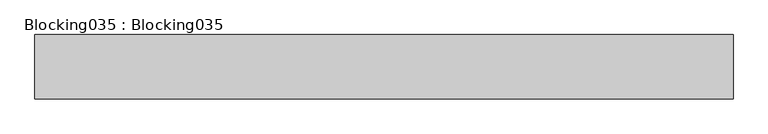
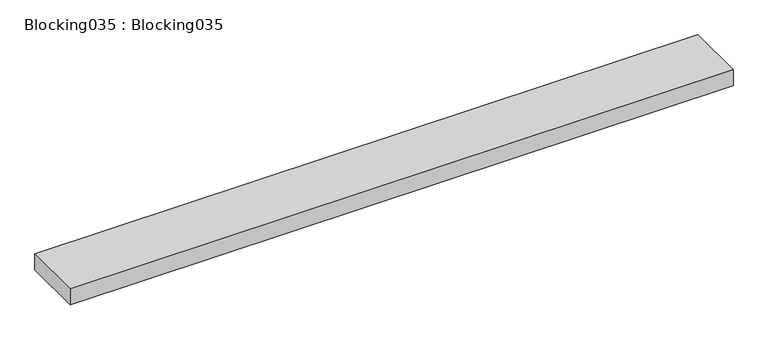
"""IFC4 building model written with IfcOpenShell, lengths in millimetres: proxy geometry, Blocking035 : Blocking035."""

from ifc_helpers import new_model, si_unit, frame, origin, place, context, project, spatial, polyline, outline, extrude, source, transform, mapped, element, save


def blocking035_blocking035_7795a8c8(model_context):
    return source(origin(), model_context, "Body", "SweptSolid", [
        extrude(outline(polyline([(3694.2883192, 10233.5057113), (3694.2883192, 10417.7246265), (5694.2883192, 10417.7246265), (5694.2883192, 10233.5057113), (3694.2883192, 10233.5057113)])), frame((0.0, 0.0, 39439.596), z_axis=(0.0, 0.0, 1.0), x_axis=(1.0, 0.0, 0.0)), (0.0, 0.0, 1.0), 50.8),
    ])


if __name__ == "__main__":
    model = new_model("IFC4")
    model_context = context("Model", 3, world=origin())
    ifc_project = project(units=[si_unit("LENGTHUNIT", "METRE", prefix="MILLI")], contexts=[model_context])
    site = spatial("IfcSite", under=ifc_project)
    building = spatial("IfcBuilding", under=site)
    placement = place(None, origin())
    blocking035_blocking035_shape = blocking035_blocking035_7795a8c8(model_context)
    element("IfcBuildingElementProxy", 1, Name="Blocking035 : Blocking035", ObjectType="Blocking035 : Blocking035", at=placement, inside=building, context=model_context, shape_type="MappedRepresentation", body=[
        mapped(blocking035_blocking035_shape, transform((0.0, 0.0, 0.0), x_axis=(1.0, 0.0, 0.0), y_axis=(0.0, 1.0, 0.0), z_axis=(0.0, 0.0, 1.0))),
    ])
    save(model, "model.ifc")

# Revit data of these elements
# Type "Blocking035 : Blocking035"
#   NameOverride = "Blocking035"
# Element 1 (IfcBuildingElementProxy, "Blocking035 : Blocking035")
#   Materials on its faces: "WOOD BLOCKING AS REQUIRED"
# Materials
#   "WOOD BLOCKING AS REQUIRED": class "Unassigned", colour RGB 166 124 85, transparency 0, Cost = 0
